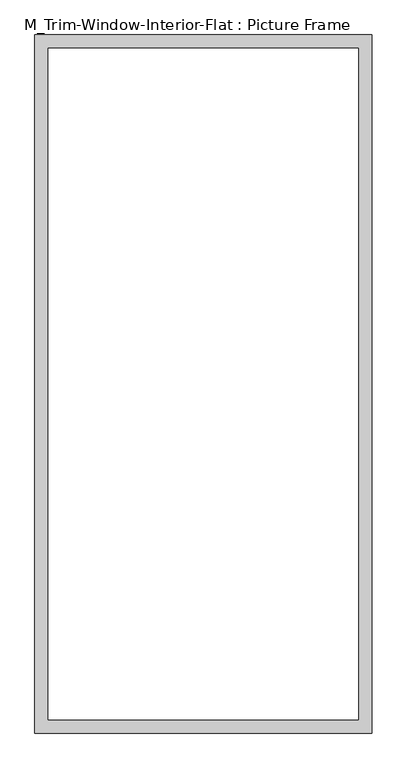
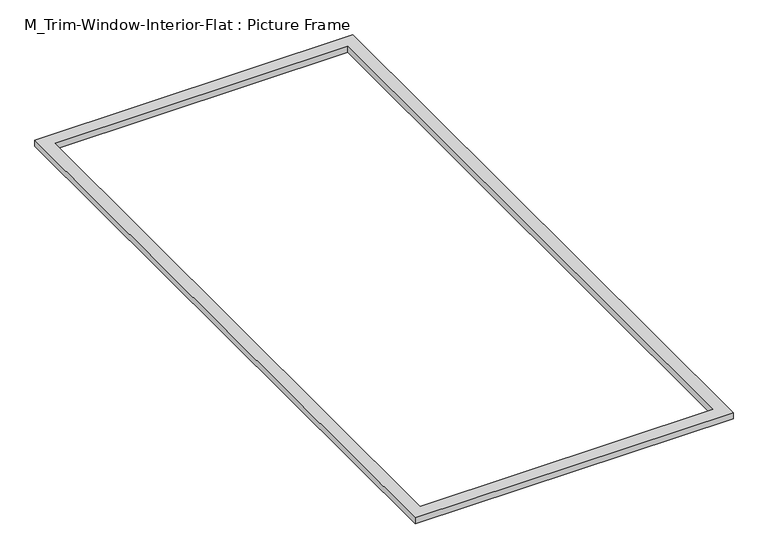
"""IFC4 building model written with IfcOpenShell, lengths in millimetres: proxy geometry, M_Trim-Window-Interior-Flat : Picture Frame."""

from ifc_helpers import new_model, si_unit, origin, origin_with_axes, place, context, project, spatial, polyline, outline, extrude, source, transform, mapped, element, save


def m_trim_window_interior_flat_picture_frame_76c67b50(model_context):
    return source(origin(), model_context, "Body", "SweptSolid", [
        extrude(outline(polyline([(747.3, -47.3), (-747.3, -47.3), (-747.3, 3047.3), (747.3, 3047.3), (747.3, -47.3)]), holes=[polyline([(687.3, 12.7), (687.3, 2987.3), (-687.3, 2987.3), (-687.3, 12.7), (687.3, 12.7)])]), origin_with_axes(), (0.0, 0.0, 1.0), 30.0),
    ])


if __name__ == "__main__":
    model = new_model("IFC4")
    model_context = context("Model", 3, world=origin())
    ifc_project = project(units=[si_unit("LENGTHUNIT", "METRE", prefix="MILLI")], contexts=[model_context])
    site = spatial("IfcSite", under=ifc_project)
    building = spatial("IfcBuilding", under=site)
    placement = place(None, origin())
    m_trim_window_interior_flat_picture_frame_shape = m_trim_window_interior_flat_picture_frame_76c67b50(model_context)
    element("IfcBuildingElementProxy", 1, Name="M_Trim-Window-Interior-Flat : Picture Frame", ObjectType="M_Trim-Window-Interior-Flat : Picture Frame", at=placement, inside=building, context=model_context, shape_type="MappedRepresentation", body=[
        mapped(m_trim_window_interior_flat_picture_frame_shape, transform((0.0, 0.0, 0.0), x_axis=(1.0, 0.0, 0.0), y_axis=(0.0, 1.0, 0.0), z_axis=(0.0, 0.0, 1.0))),
    ])
    save(model, "model.ifc")

# Revit data of these elements
# Type "M_Trim-Window-Interior-Flat : Picture Frame"
#   Trim Thickness_Picture Frame = 30 mm
#   Trim Width = 60 mm
#   Trim Thickness_with Sill = 20 mm
#   Sill Thickness = 30 mm
#   Opening Width [instance default] = 600 mm
#   Opening Height [instance default] = 900 mm
#   Default Elevation = 1200 mm
#   Sill = no
#   Picture Frame = yes
#   Trim Material [instance default] = none
# Element 1 (IfcBuildingElementProxy, "M_Trim-Window-Interior-Flat : Picture Frame")
#   Opening Width = 1400 mm
#   Opening Height = 3000 mm
#   Trim Material = Wood - Stained
#   Materials on its faces: "Wood - Stained"
# Materials
#   "Wood - Stained": class "Wood", colour RGB 173 132 96, transparency 0, Cost = 0
